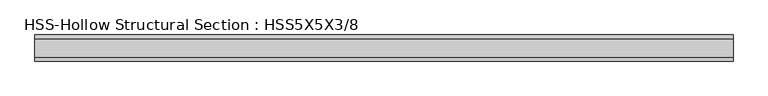
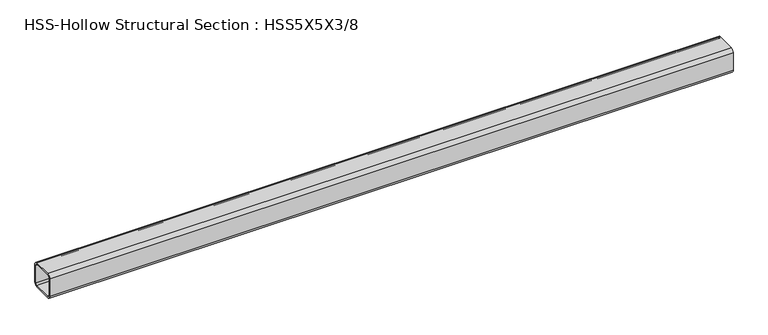
"""IFC4 building model written with IfcOpenShell, lengths in millimetres: member geometry, HSS-Hollow Structural Section : HSS5X5X3/8."""

import ifcopenshell
import ifcopenshell.guid

model = None  # the IFC model being written
_history = None  # IfcOwnerHistory: only IFC2X3 demands one
_inside = {}  # id of a spatial element -> (the spatial element, [elements in it])
_under = {}  # id of a project, library or spatial element -> (it, [spatial elements below it])
_declared = {}  # id of a project -> (the project, [libraries it declares])
_typed = {}  # id of a type object -> (the type object, [elements of that type])
_made_of = {}  # id of a material, layer set ... -> (it, [elements and type objects made of it])


def new_model(schema):
    """Start an empty IFC model of exactly this schema.

    Asked for "IFC4X3", IfcOpenShell would pick the latest addendum, in which some entities
    have other attributes; the version numbers below select the first issue.
    IFC2X3 requires an IfcOwnerHistory on every rooted entity: one is made here for all.
    """
    global model, _history
    if schema == "IFC4X3":
        model = ifcopenshell.file(schema_version=(4, 3, 0, 0))
    else:
        model = ifcopenshell.file(schema=schema)
    _inside.clear()
    _under.clear()
    _declared.clear()
    _typed.clear()
    _made_of.clear()
    _history = None
    if model.schema == "IFC2X3":
        org = make("IfcOrganization", Name="unknown")
        user = make(
            "IfcPersonAndOrganization",
            ThePerson=make("IfcPerson", FamilyName="unknown"),
            TheOrganization=org,
        )
        app = make(
            "IfcApplication",
            ApplicationDeveloper=org,
            Version="unknown",
            ApplicationFullName="unknown",
            ApplicationIdentifier="unknown",
        )
        _history = make(
            "IfcOwnerHistory",
            OwningUser=user,
            OwningApplication=app,
            ChangeAction="ADDED",
            CreationDate=0,
        )
    return model


def make(cls, **values):
    """One entity of the class cls with the attributes given. An attribute that is None is left unset."""
    return model.create_entity(
        cls, **{name: value for name, value in values.items() if value is not None}
    )


def rooted(cls, **values):
    """An entity with a GlobalId (a new one), such as an element, a storey or a relation."""
    return make(cls, GlobalId=ifcopenshell.guid.new(), OwnerHistory=_history, **values)


def si_unit(unit_type, name, prefix=None):
    """IfcSIUnit, for example si_unit("LENGTHUNIT", "METRE", prefix="MILLI")."""
    return make("IfcSIUnit", UnitType=unit_type, Prefix=prefix, Name=name)


def assignment(units):
    """IfcUnitAssignment: the units of a project."""
    return None if units is None else make("IfcUnitAssignment", Units=units)


def point(xyz):
    """IfcCartesianPoint."""
    return None if xyz is None else make("IfcCartesianPoint", Coordinates=xyz)


def direction(xyz):
    """IfcDirection."""
    return None if xyz is None else make("IfcDirection", DirectionRatios=xyz)


def frame(location, z_axis=None, x_axis=None):
    """IfcAxis2Placement3D, a coordinate frame: its origin and axes. An axis left out is left unset."""
    return make(
        "IfcAxis2Placement3D",
        Location=point(location),
        Axis=direction(z_axis),
        RefDirection=direction(x_axis),
    )


def frame_2d(location, x_axis=None):
    """IfcAxis2Placement2D, a coordinate frame in the plane: its origin and x axis."""
    return make(
        "IfcAxis2Placement2D", Location=point(location), RefDirection=direction(x_axis)
    )


def origin():
    """The frame at (0, 0, 0) with its axes left unset."""
    return frame((0.0, 0.0, 0.0))


def place(relative_to, where):
    """IfcLocalPlacement: puts the frame where relative to a parent placement (None: the world)."""
    return make(
        "IfcLocalPlacement", PlacementRelTo=relative_to, RelativePlacement=where
    )


def context(
    kind, dimensions, precision=None, world=None, true_north=None, identifier=None
):
    """IfcGeometricRepresentationContext, for example the 3D "Model" context."""
    return make(
        "IfcGeometricRepresentationContext",
        ContextIdentifier=identifier,
        ContextType=kind,
        CoordinateSpaceDimension=dimensions,
        Precision=precision,
        WorldCoordinateSystem=world,
        TrueNorth=true_north,
    )


def project(units=None, contexts=None):
    """IfcProject with its units and contexts."""
    return rooted(
        "IfcProject",
        Name="project",
        RepresentationContexts=contexts,
        UnitsInContext=assignment(units),
    )


def spatial(cls, under=None, at=None, **own):
    """A site, building, storey or space (cls), placed at a placement, below another one or the project."""
    s = rooted(cls, ObjectPlacement=at, **own)
    if under is not None:
        _under.setdefault(under.id(), (under, []))[1].append(s)
    return s


def polyline(points):
    """IfcPolyline through the points."""
    return make("IfcPolyline", Points=[point(p) for p in points])


def circle_curve(where, radius):
    """IfcCircle in the frame where."""
    return make("IfcCircle", Position=where, Radius=radius)


def trimmed(basis, trim1, trim2, sense, master):
    """IfcTrimmedCurve: the piece of a basis curve between two trims."""
    return make(
        "IfcTrimmedCurve",
        BasisCurve=basis,
        Trim1=trim1,
        Trim2=trim2,
        SenseAgreement=sense,
        MasterRepresentation=master,
    )


def segment(curve, same_sense, transition):
    """IfcCompositeCurveSegment."""
    return make(
        "IfcCompositeCurveSegment",
        Transition=transition,
        SameSense=same_sense,
        ParentCurve=curve,
    )


def composite_curve(segments, self_intersect=None):
    """IfcCompositeCurve: segments joined end to end."""
    return make("IfcCompositeCurve", Segments=segments, SelfIntersect=self_intersect)


def outline(outer, holes=None, kind="AREA"):
    """IfcArbitraryClosedProfileDef: a profile drawn as a closed curve; with holes, ...WithVoids."""
    if holes is None:
        return make("IfcArbitraryClosedProfileDef", ProfileType=kind, OuterCurve=outer)
    return make(
        "IfcArbitraryProfileDefWithVoids",
        ProfileType=kind,
        OuterCurve=outer,
        InnerCurves=holes,
    )


def extrude(swept, where, along, depth):
    """IfcExtrudedAreaSolid: the profile swept, set in the frame where, extruded along a direction by depth."""
    return make(
        "IfcExtrudedAreaSolid",
        SweptArea=swept,
        Position=where,
        ExtrudedDirection=direction(along),
        Depth=depth,
    )


def shape(context_of_items, identifier, shape_type, items):
    """IfcShapeRepresentation: the items that make up one representation, for example the "Body"."""
    return make(
        "IfcShapeRepresentation",
        ContextOfItems=context_of_items,
        RepresentationIdentifier=identifier,
        RepresentationType=shape_type,
        Items=items,
    )


def source(mapping_origin, context_of_items, identifier, shape_type, items):
    """IfcRepresentationMap: a shape defined once, which mapped items show again and again."""
    return make(
        "IfcRepresentationMap",
        MappingOrigin=mapping_origin,
        MappedRepresentation=shape(context_of_items, identifier, shape_type, items),
    )


def transform(
    local_origin,
    x_axis=None,
    y_axis=None,
    z_axis=None,
    scale=None,
    scale2=None,
    scale3=None,
    uniform=True,
):
    """IfcCartesianTransformationOperator3D, or its non-uniform kind. x_axis, y_axis, z_axis: its Axis1, 2, 3."""
    if uniform:
        return make(
            "IfcCartesianTransformationOperator3D",
            Axis1=direction(x_axis),
            Axis2=direction(y_axis),
            LocalOrigin=point(local_origin),
            Scale=scale,
            Axis3=direction(z_axis),
        )
    return make(
        "IfcCartesianTransformationOperator3DnonUniform",
        Axis1=direction(x_axis),
        Axis2=direction(y_axis),
        LocalOrigin=point(local_origin),
        Scale=scale,
        Axis3=direction(z_axis),
        Scale2=scale2,
        Scale3=scale3,
    )


def mapped(mapping_source, mapping_target):
    """IfcMappedItem: shows the shape of a source again, moved by a transform."""
    return make(
        "IfcMappedItem", MappingSource=mapping_source, MappingTarget=mapping_target
    )


def made_of(thing, what):
    """Note that an element or type object is made of a material, layer set ...; save() writes the relation."""
    if what is not None:
        _made_of.setdefault(what.id(), (what, []))[1].append(thing)
    return thing


def element(
    cls,
    number,
    at=None,
    inside=None,
    cuts=None,
    type_object=None,
    material=None,
    context=None,
    identifier="Body",
    shape_type=None,
    held_by="IfcProductDefinitionShape",
    body=None,
    shapes=None,
    **own,
):
    """One element of the class cls, such as IfcWall. Its Tag is "e" and its number.

    at: its placement. inside: the storey or other place that contains it. cuts: it is an
    opening in that element (IfcRelVoidsElement). A single representation is given by context,
    identifier, shape_type and body (its items); several are given by shapes. held_by: the class
    of the entity that holds the representations. save() writes the other relations.
    """
    e = rooted(cls, Tag="e%d" % number, ObjectPlacement=at, **own)
    if body is not None:
        shapes = [shape(context, identifier, shape_type, body)]
    if shapes is not None:
        e.Representation = make(held_by, Representations=shapes)
    if inside is not None:
        _inside.setdefault(inside.id(), (inside, []))[1].append(e)
    if cuts is not None:
        rooted(
            "IfcRelVoidsElement", RelatingBuildingElement=cuts, RelatedOpeningElement=e
        )
    if type_object is not None:
        _typed.setdefault(type_object.id(), (type_object, []))[1].append(e)
    return made_of(e, material)


def aggregate(whole, parts):
    """IfcRelAggregates: a whole, such as a stair, and the parts it consists of."""
    return rooted("IfcRelAggregates", RelatingObject=whole, RelatedObjects=parts)


def save(model, path):
    """Write the relations noted so far, then the file.

    IfcRelAggregates (storeys below a building ...), IfcRelContainedInSpatialStructure (elements
    in a storey), IfcRelDefinesByType, IfcRelAssociatesMaterial and IfcRelDeclares: one each for
    every whole, place, type object, material and project.
    """
    for whole, parts in _under.values():
        aggregate(whole, parts)
    for where, things in _inside.values():
        rooted(
            "IfcRelContainedInSpatialStructure",
            RelatedElements=things,
            RelatingStructure=where,
        )
    for kind, things in _typed.values():
        rooted("IfcRelDefinesByType", RelatedObjects=things, RelatingType=kind)
    for what, things in _made_of.values():
        rooted("IfcRelAssociatesMaterial", RelatedObjects=things, RelatingMaterial=what)
    for by, libraries in _declared.values():
        rooted("IfcRelDeclares", RelatingContext=by, RelatedDefinitions=libraries)
    model.write(path)


def hss_hollow_structural_section_hss5x5x3_8_6dea9a89(model_context):
    return source(origin(), model_context, "Body", "SweptSolid", [
        extrude(outline(composite_curve([segment(polyline([(63.5, 45.7708), (63.5, -45.7708)]), True, "CONTINUOUS"), segment(trimmed(circle_curve(frame_2d((45.7708, -45.7708)), 17.7292), [point((63.5, -45.7708))], [point((45.7708, -63.5))], False, "CARTESIAN"), True, "CONTINUOUS"), segment(polyline([(45.7708, -63.5), (-45.7708, -63.5)]), True, "CONTINUOUS"), segment(trimmed(circle_curve(frame_2d((-45.7708, -45.7708)), 17.7292), [point((-45.7708, -63.5))], [point((-63.5, -45.7708))], False, "CARTESIAN"), True, "CONTINUOUS"), segment(polyline([(-63.5, -45.7708), (-63.5, 45.7708)]), True, "CONTINUOUS"), segment(trimmed(circle_curve(frame_2d((-45.7708, 45.7708)), 17.7292), [point((-63.5, 45.7708))], [point((-45.7708, 63.5))], False, "CARTESIAN"), True, "CONTINUOUS"), segment(polyline([(-45.7708, 63.5), (45.7708, 63.5)]), True, "CONTINUOUS"), segment(trimmed(circle_curve(frame_2d((45.7708, 45.7708)), 17.7292), [point((45.7708, 63.5))], [point((63.5, 45.7708))], False, "CARTESIAN"), True, "CONTINUOUS")], self_intersect=False), holes=[composite_curve([segment(trimmed(circle_curve(frame_2d((-45.7708, 45.7708)), 8.8646), [point((-45.7708, 54.6354))], [point((-54.6354, 45.7708))], True, "CARTESIAN"), True, "CONTINUOUS"), segment(polyline([(-54.6354, 45.7708), (-54.6354, -45.7708)]), True, "CONTINUOUS"), segment(trimmed(circle_curve(frame_2d((-45.7708, -45.7708)), 8.8646), [point((-54.6354, -45.7708))], [point((-45.7708, -54.6354))], True, "CARTESIAN"), True, "CONTINUOUS"), segment(polyline([(-45.7708, -54.6354), (45.7708, -54.6354)]), True, "CONTINUOUS"), segment(trimmed(circle_curve(frame_2d((45.7708, -45.7708)), 8.8646), [point((45.7708, -54.6354))], [point((54.6354, -45.7708))], True, "CARTESIAN"), True, "CONTINUOUS"), segment(polyline([(54.6354, -45.7708), (54.6354, 45.7708)]), True, "CONTINUOUS"), segment(trimmed(circle_curve(frame_2d((45.7708, 45.7708)), 8.8646), [point((54.6354, 45.7708))], [point((45.7708, 54.6354))], True, "CARTESIAN"), True, "CONTINUOUS"), segment(polyline([(45.7708, 54.6354), (-45.7708, 54.6354)]), True, "CONTINUOUS")], self_intersect=False)]), frame((-1658.4224836, 0.0, 0.0), z_axis=(1.0, 0.0, 0.0), x_axis=(0.0, 1.0, 0.0)), (0.0, 0.0, 1.0), 3392.5854856),
    ])


if __name__ == "__main__":
    model = new_model("IFC4")
    model_context = context("Model", 3, world=origin())
    ifc_project = project(units=[si_unit("LENGTHUNIT", "METRE", prefix="MILLI")], contexts=[model_context])
    site = spatial("IfcSite", under=ifc_project)
    building = spatial("IfcBuilding", under=site)
    placement = place(None, origin())
    hss_hollow_structural_section_hss5x5x3_8_shape = hss_hollow_structural_section_hss5x5x3_8_6dea9a89(model_context)
    element("IfcMember", 1, ObjectType="HSS-Hollow Structural Section : HSS5X5X3/8", at=placement, inside=building, context=model_context, shape_type="MappedRepresentation", body=[
        mapped(hss_hollow_structural_section_hss5x5x3_8_shape, transform((0.0, 0.0, 0.0), x_axis=(1.0, 0.0, 0.0), y_axis=(0.0, 1.0, 0.0), z_axis=(0.0, 0.0, 1.0))),
    ])
    save(model, "model.ifc")

# Revit data of these elements
# Type "HSS-Hollow Structural Section : HSS5X5X3/8"
#   Assembly Code = "B10"
#   Shape = "Square"
#   W = 22.3
#   Ht = 0' - 5"
#   Length [instance default] = 5' - 0"
#   b = 0' - 5"
#   kr = 0' - 0.698"
#   t = 0' - 0.349"
#   A = 0.0429167 SF
#   Structural Material [instance default] = Steel ASTM A500, Grade B, Rectangular and Square
# Element 1 (IfcMember, "HSS-Hollow Structural Section : HSS5X5X3/8")
#   Materials on its faces: "Steel ASTM A500, Grade B, Rectangular and Square"
# Materials
#   "Steel ASTM A500, Grade B, Rectangular and Square": class "Metal", colour RGB 199 199 199, transparency 0, Description = "Carbon steel", Cost = 0
